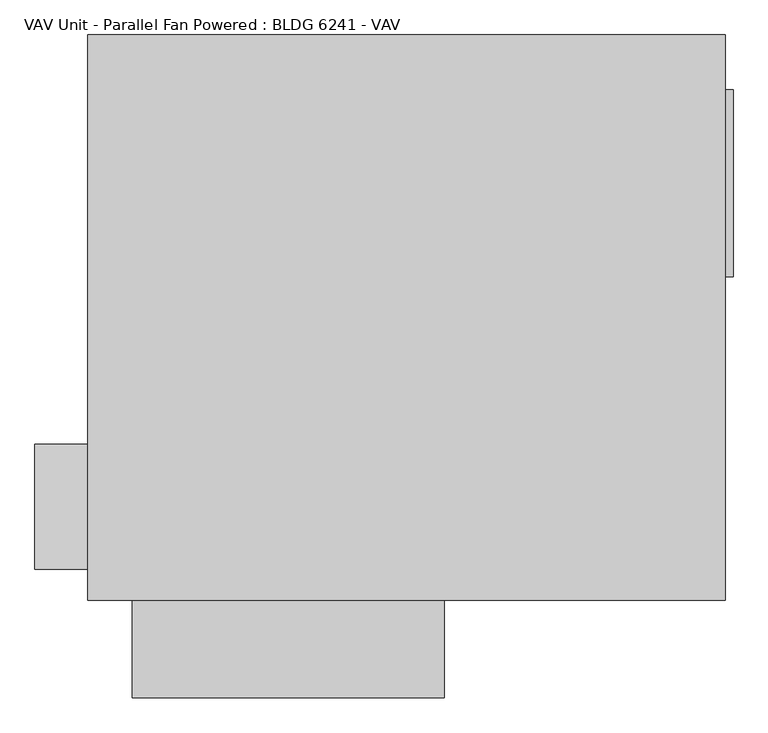
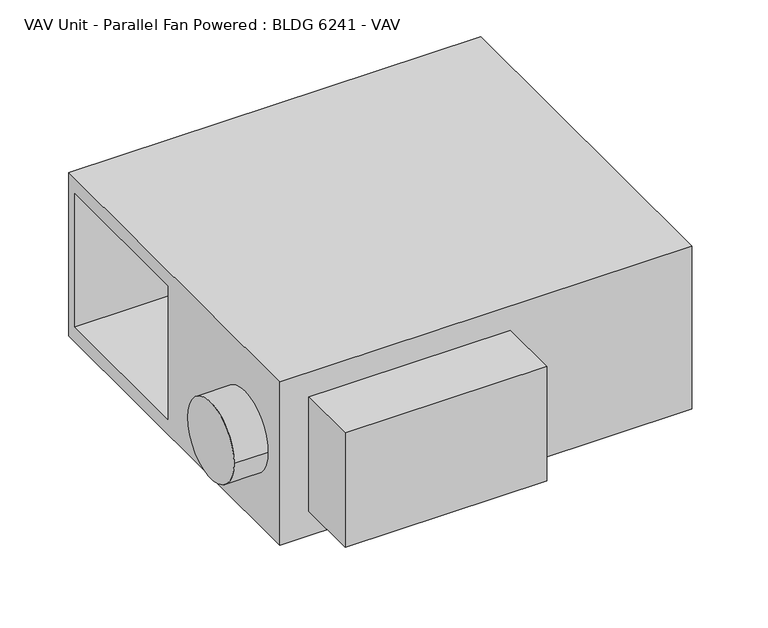
"""IFC4 building model written with IfcOpenShell, lengths in millimetres: proxy geometry, VAV Unit - Parallel Fan Powered : BLDG 6241 - VAV."""

from ifc_helpers import new_model, si_unit, point, frame, frame_2d, origin, place, context, project, spatial, polyline, circle_curve, trimmed, segment, composite_curve, outline, extrude, faceted_brep, source, transform, mapped, element, save


def vav_unit_parallel_fan_powered_bldg_6241_vav_9e34d673(model_context):
    return source(origin(), model_context, "Body", "SolidModel", [
        extrude(outline(polyline([(531.8125, 66.675), (519.1125, 66.675), (519.1125, 371.475), (531.8125, 371.475), (531.8125, 66.675)])), frame((0.0, 0.0, -139.7), z_axis=(0.0, 0.0, 1.0), x_axis=(1.0, 0.0, 0.0)), (0.0, 0.0, 1.0), 279.4),
        extrude(outline(polyline([(61.9125, -460.375), (61.9125, -619.125), (-446.0875, -619.125), (-446.0875, -460.375), (61.9125, -460.375)])), frame((0.0, 0.0, -152.4), z_axis=(0.0, 0.0, 1.0), x_axis=(1.0, 0.0, 0.0)), (0.0, 0.0, 1.0), 304.8),
        extrude(outline(composite_curve([segment(trimmed(circle_curve(frame_2d((-307.975, 0.0)), 101.6), [point((-206.375, 0.0))], [point((-409.575, 0.0))], False, "CARTESIAN"), True, "CONTINUOUS"), segment(trimmed(circle_curve(frame_2d((-307.975, 0.0)), 101.6), [point((-409.575, 0.0))], [point((-206.375, 0.0))], False, "CARTESIAN"), True, "CONTINUOUS")], self_intersect=False)), frame((-604.8375, 0.0, 0.0), z_axis=(1.0, 0.0, 0.0), x_axis=(0.0, 1.0, 0.0)), (0.0, 0.0, 1.0), 85.725),
        faceted_brep([(519.1125, -460.375, 217.4875), (519.1125, 460.375, 217.4875), (-519.1125, 460.375, 217.4875), (-519.1125, -460.375, 217.4875), (519.1125, -460.375, -217.4875), (-519.1125, -460.375, -217.4875), (-519.1125, 460.375, -217.4875), (519.1125, 460.375, -217.4875), (-519.1125, 434.975, 177.8), (-519.1125, 28.575, 177.8), (-519.1125, 28.575, -177.8), (-519.1125, 434.975, -177.8), (0.0, 434.975, 177.8), (0.0, 434.975, -177.8), (0.0, 28.575, -177.8), (0.0, 28.575, 177.8)], [[[0, 1, 2, 3]], [[4, 5, 6, 7]], [[3, 5, 4, 0]], [[2, 6, 5, 3], [8, 9, 10, 11]], [[1, 7, 6, 2]], [[0, 4, 7, 1]], [[12, 13, 14, 15]], [[12, 8, 11, 13]], [[13, 11, 10, 14]], [[14, 10, 9, 15]], [[15, 9, 8, 12]]]),
    ])


if __name__ == "__main__":
    model = new_model("IFC4")
    model_context = context("Model", 3, world=origin())
    ifc_project = project(units=[si_unit("LENGTHUNIT", "METRE", prefix="MILLI")], contexts=[model_context])
    site = spatial("IfcSite", under=ifc_project)
    building = spatial("IfcBuilding", under=site)
    placement = place(None, origin())
    vav_unit_parallel_fan_powered_bldg_6241_vav_shape = vav_unit_parallel_fan_powered_bldg_6241_vav_9e34d673(model_context)
    element("IfcBuildingElementProxy", 1, Name="VAV Unit - Parallel Fan Powered : BLDG 6241 - VAV", ObjectType="VAV Unit - Parallel Fan Powered : BLDG 6241 - VAV", at=placement, inside=building, context=model_context, shape_type="MappedRepresentation", body=[
        mapped(vav_unit_parallel_fan_powered_bldg_6241_vav_shape, transform((0.0, 0.0, 0.0), x_axis=(1.0, 0.0, 0.0), y_axis=(0.0, 1.0, 0.0), z_axis=(0.0, 0.0, 1.0))),
    ])
    save(model, "model.ifc")

# Revit data of these elements
# Type "VAV Unit - Parallel Fan Powered : BLDG 6241 - VAV"
#   Width2 = 1' - 0"
#   Voltage = 120 V
#   UnitWidth = 3' - 4 7/8"
#   UnitHeight = 3' - 0 1/4"
#   UnitDepth = 1' - 5 1/8"
#   SupplyConnectorWidth = 1' - 0"
#   SupplyConnectorVerticalOffset = 0' - 2 1/8"
#   SupplyConnectorLength = 0' - 0 1/2"
#   SupplyConnectorHorizontalOffset = 0' - 3 1/2"
#   SupplyConnectorDepth = 0' - 11"
#   SupplyAirConnectorCenterOffset = 0' - 9 1/2"
#   PrimaryToSupplyRatio [instance default] = 0.2
#   PrimaryAirOffset = 0' - 6"
#   PrimaryAirFlow [instance default] = 180 CFM
#   PrimaryAirConnectorVerticalOffset = 0' - 8 9/16"
#   PrimaryAirConnectorRadius = 0' - 4"
#   PrimaryAirConnectorLength = 0' - 3 3/8"
#   PrimaryAirConnectorDiameter = 0' - 8"
#   PrimaryAirConnectorCenterOffset = 0' - 6"
#   Pressure Drop [instance default] = 0.02 in-wg
#   InducedAirInletWidth = 1' - 4"
#   InducedAirInletDepth = 1' - 2"
#   InducedAirConnectorHorizontalOffset = 0' - 1"
#   InducedAirConnectorCenterOffset = 0' - 9"
#   Height2 = 0' - 11"
#   ElectricalConnectionBoxWidth = 1' - 8"
#   ElectricalConnectionBoxOffset = 0' - 2 7/8"
#   ElectricalConnectionBoxHeight = 0' - 6 1/4"
#   ElectricalConnectionBoxDepth = 1' - 0"
#   SupplyAirFlow [instance default] = 900 CFM
#   Apparent Load = 271 VA
#   SupplyAirConnectorIndex = 2
#   PrimaryAirConnectorIndex = 1
#   Number of Poles = 1
#   InducedAirConnectorIndex = 3
#   VAV Material = none
#   Load Classification = Cooling
#   Default Elevation = 0
#   Assembly Code = ""
